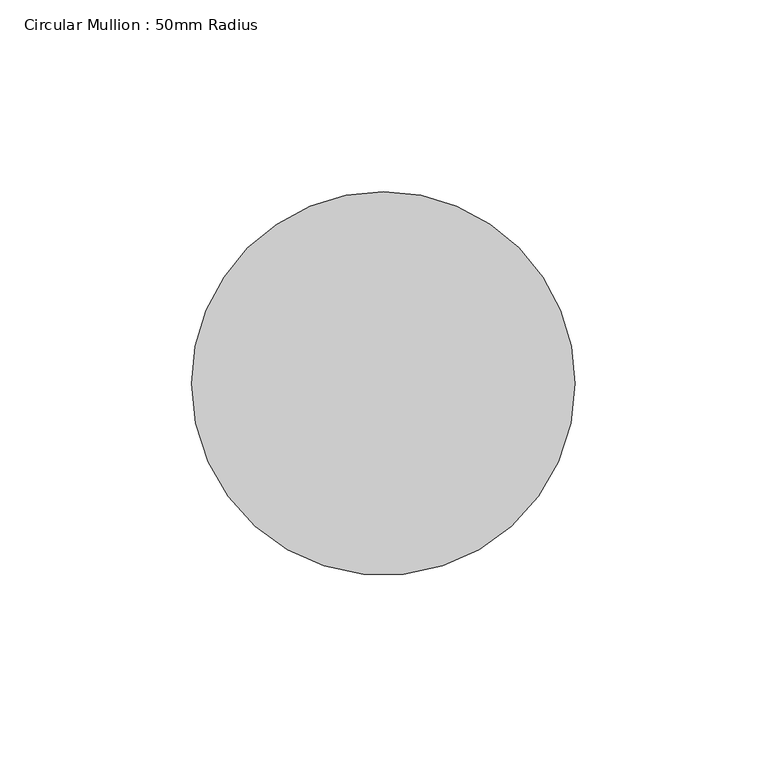
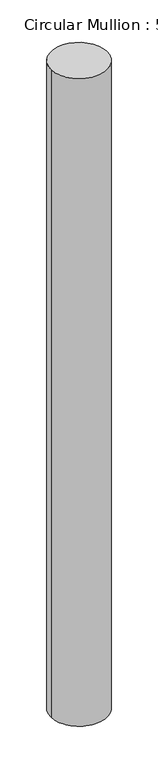
"""IFC4 building model written with IfcOpenShell, lengths in millimetres: member geometry, Circular Mullion : 50mm Radius."""

from ifc_helpers import new_model, si_unit, frame, origin, place, context, project, spatial, circle_curve, ellipse_curve, source, transform, mapped, element, save
from ifc_brep_helpers import plane_surface, cylinder_surface, advanced_brep


def circular_mullion_50mm_radius_5d5aa93d(model_context):
    return source(origin(), model_context, "Body", "AdvancedBrep", [
        advanced_brep(
        [(0.0, 0.0, -1225.3294255), (-100.0, 0.0, -1225.3294255), (-100.0, 0.0, 0.6461643), (0.0, 0.0, 0.0)],
        [
            (0, 1, circle_curve(frame((-50.0, 0.0, -1225.3294255), z_axis=(0.0, 0.0, -1.0), x_axis=(1.0, 0.0, 0.0)), 50.0)),
            (1, 0, circle_curve(frame((-50.0, 0.0, -1225.3294255), z_axis=(0.0, 0.0, -1.0), x_axis=(1.0, 0.0, 0.0)), 50.0)),
            (2, 3, ellipse_curve(frame((-50.0, 0.0, 0.3230821), z_axis=(-0.006460988484777742, -0.012678916618819999, -0.9998987452243215), x_axis=(-0.453986803032295, -0.8908947656001178, 0.014230224834036081)), 50.0050633, 50.0)),
            (3, 0),
            (1, 2),
            (3, 2, ellipse_curve(frame((-50.0, 0.0, 0.3230821), z_axis=(-0.006460988484777742, -0.012678916618819999, -0.9998987452243215), x_axis=(-0.453986803032295, -0.8908947656001178, 0.014230224834036081)), 50.0050633, 50.0)),
        ],
        [
            plane_surface(frame((0.0, -100.0, -1225.3294255), z_axis=(0.0, 0.0, -1.0), x_axis=(-1.0, 0.0, 0.0))),
            cylinder_surface(frame((-50.0, 0.0, 0.0), z_axis=(0.0, 0.0, 1.0), x_axis=(1.0, 0.0, 0.0)), 50.0),
            plane_surface(frame((-271.5722225, 138.3891901, 0.0), z_axis=(0.006460988484777744, 0.012678916618820002, 0.9998987452243218), x_axis=(0.4539868030322946, 0.890894765600118, -0.014230224834043228))),
        ],
        [
            (0, [[1, 2]]),
            (1, [[3, 4, -2, 5]]),
            (1, [[6, -5, -1, -4]]),
            (2, [[-3, -6]]),
        ],
    ),
    ])


if __name__ == "__main__":
    model = new_model("IFC4")
    model_context = context("Model", 3, world=origin())
    ifc_project = project(units=[si_unit("LENGTHUNIT", "METRE", prefix="MILLI")], contexts=[model_context])
    site = spatial("IfcSite", under=ifc_project)
    building = spatial("IfcBuilding", under=site)
    placement = place(None, origin())
    circular_mullion_50mm_radius_shape = circular_mullion_50mm_radius_5d5aa93d(model_context)
    element("IfcMember", 1, ObjectType="Circular Mullion : 50mm Radius", at=placement, inside=building, context=model_context, shape_type="MappedRepresentation", body=[
        mapped(circular_mullion_50mm_radius_shape, transform((0.0, 0.0, 0.0), x_axis=(1.0, 0.0, 0.0), y_axis=(0.0, 1.0, 0.0), z_axis=(0.0, 0.0, 1.0))),
    ])
    save(model, "model.ifc")

# Revit data of these elements
# Type "Circular Mullion : 50mm Radius"
#   built-in parameter 1007350 = 0.164042 (stored number, unit not read)
# Element 1 (IfcMember, "Circular Mullion : 50mm Radius")
#   Materials on its faces: "Aluminium"
# Materials
#   "Aluminium": class "Metal", colour RGB 247 247 247, transparency 0, Description = "Aluminium 6061", Cost = 0
